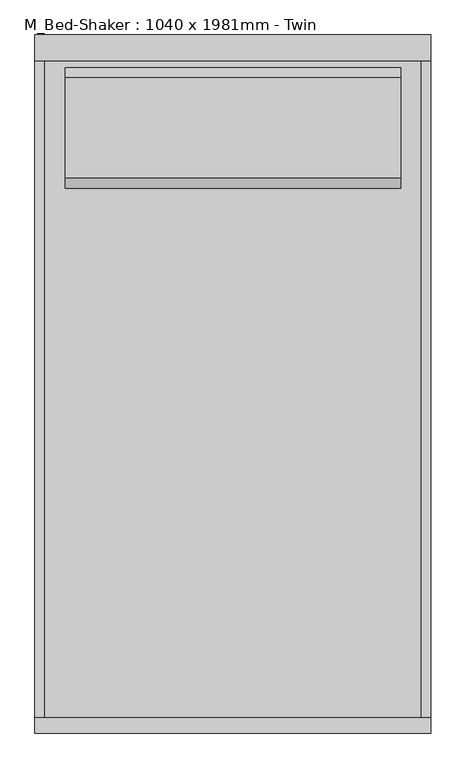
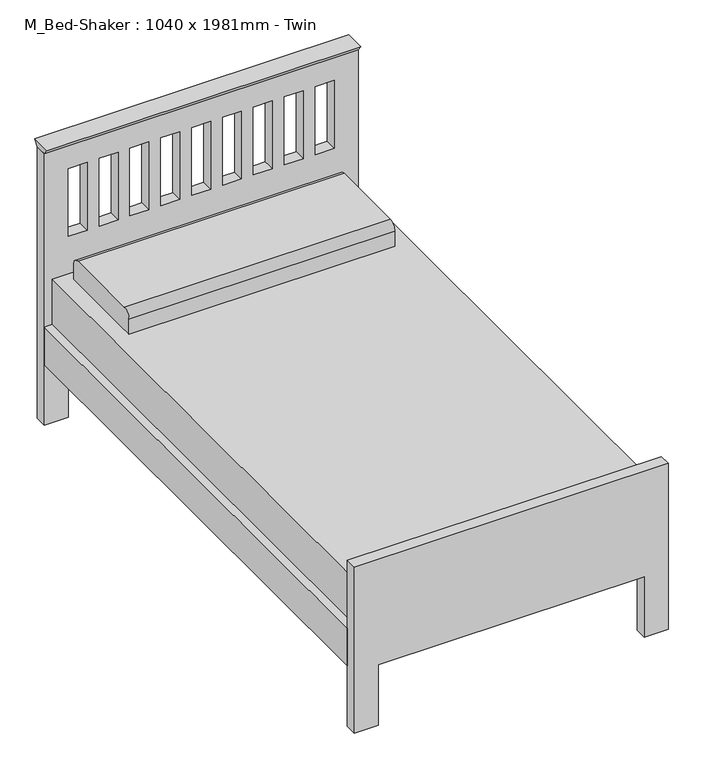
"""IFC4 building model written with IfcOpenShell, lengths in millimetres: furniture geometry, M_Bed-Shaker : 1040 x 1981mm - Twin."""

from ifc_helpers import new_model, si_unit, point, frame, frame_2d, origin, place, context, project, spatial, polyline, circle_curve, trimmed, segment, composite_curve, outline, extrude, source, transform, mapped, element, save


def m_bed_shaker_1040_x_1981mm_twin_8a9c4475(model_context):
    return source(origin(), model_context, "Body", "SweptSolid", [
        extrude(outline(polyline([(-38.1, 914.4), (-51.9545455, 933.45), (13.8545455, 933.45), (0.0, 914.4), (-38.1, 914.4)])), frame((-518.8365546, 0.0, 0.0), z_axis=(1.0, 0.0, 0.0), x_axis=(0.0, 1.0, 0.0)), (0.0, 0.0, 1.0), 1000.0533613),
        extrude(outline(composite_curve([segment(polyline([(-373.2486637, 482.6), (-373.2486637, 533.4)]), True, "CONTINUOUS"), segment(trimmed(circle_curve(frame_2d((-347.8486637, 533.4)), 25.4), [point((-373.2486637, 533.4))], [point((-347.8486637, 558.8))], False, "CARTESIAN"), True, "CONTINUOUS"), segment(polyline([(-347.8486637, 558.8), (-93.8486637, 558.8)]), True, "CONTINUOUS"), segment(trimmed(circle_curve(frame_2d((-93.8486637, 533.4)), 25.4), [point((-93.8486637, 558.8))], [point((-68.4486637, 533.4))], False, "CARTESIAN"), True, "CONTINUOUS"), segment(polyline([(-68.4486637, 533.4), (-68.4486637, 482.6), (-373.2486637, 482.6)]), True, "CONTINUOUS")], self_intersect=False)), frame((-442.85, 0.0, 0.0), z_axis=(1.0, 0.0, 0.0), x_axis=(0.0, 1.0, 0.0)), (0.0, 0.0, 1.0), 847.6),
        extrude(outline(polyline([(455.55, -38.1), (455.55, -1711.9), (-493.65, -1711.9), (-493.65, -38.1), (455.55, -38.1)])), frame((0.0, 0.0, 228.6), z_axis=(0.0, 0.0, 1.0), x_axis=(1.0, 0.0, 0.0)), (0.0, 0.0, 1.0), 254.0),
        extrude(outline(polyline([(455.55, -1711.9), (455.55, -38.1), (480.95, -38.1), (480.95, -1711.9), (455.55, -1711.9)])), frame((0.0, 0.0, 203.0994861), z_axis=(0.0, 0.0, 1.0), x_axis=(1.0, 0.0, 0.0)), (0.0, 0.0, 1.0), 127.0),
        extrude(outline(polyline([(-519.05, -1711.9), (-519.05, -38.1), (-493.65, -38.1), (-493.65, -1711.9), (-519.05, -1711.9)])), frame((0.0, 0.0, 203.5755296), z_axis=(0.0, 0.0, 1.0), x_axis=(1.0, 0.0, 0.0)), (0.0, 0.0, 1.0), 127.0),
        extrude(outline(polyline([(0.0, -442.85), (203.2, -442.85), (203.2, 404.75), (0.0, 404.75), (0.0, 480.95), (558.8, 480.95), (558.8, -519.05), (0.0, -519.05), (0.0, -442.85)])), frame((0.0, -1750.0, 0.0), z_axis=(0.0, 1.0, 0.0), x_axis=(0.0, 0.0, 1.0)), (0.0, 0.0, 1.0), 38.1),
        extrude(outline(polyline([(914.4, 481.2168067), (914.4, -518.8365546), (0.0, -518.8365546), (0.0, -442.85), (203.2, -442.85), (203.2, 404.75), (0.0, 404.75), (0.0, 481.2168067), (914.4, 481.2168067)]), holes=[polyline([(838.2, -382.5388889), (609.6, -382.5388889), (609.6, -442.85), (838.2, -442.85), (838.2, -382.5388889)]), polyline([(838.2, -284.1277778), (609.6, -284.1277778), (609.6, -344.4388889), (838.2, -344.4388889), (838.2, -284.1277778)]), polyline([(838.2, -185.7166667), (609.6, -185.7166667), (609.6, -246.0277778), (838.2, -246.0277778), (838.2, -185.7166667)]), polyline([(838.2, -87.3055556), (609.6, -87.3055556), (609.6, -147.6166667), (838.2, -147.6166667), (838.2, -87.3055556)]), polyline([(838.2, 109.5166667), (609.6, 109.5166667), (609.6, 49.2055556), (838.2, 49.2055556), (838.2, 109.5166667)]), polyline([(838.2, 207.9277778), (609.6, 207.9277778), (609.6, 147.6166667), (838.2, 147.6166667), (838.2, 207.9277778)]), polyline([(838.2, 306.3388889), (609.6, 306.3388889), (609.6, 246.0277778), (838.2, 246.0277778), (838.2, 306.3388889)]), polyline([(838.2, 404.75), (609.6, 404.75), (609.6, 344.4388889), (838.2, 344.4388889), (838.2, 404.75)]), polyline([(838.2, 11.1055556), (609.6, 11.1055556), (609.6, -49.2055556), (838.2, -49.2055556), (838.2, 11.1055556)])]), frame((0.0, -38.1, 0.0), z_axis=(0.0, 1.0, 0.0), x_axis=(0.0, 0.0, 1.0)), (0.0, 0.0, 1.0), 38.1),
    ])


if __name__ == "__main__":
    model = new_model("IFC4")
    model_context = context("Model", 3, world=origin())
    ifc_project = project(units=[si_unit("LENGTHUNIT", "METRE", prefix="MILLI")], contexts=[model_context])
    site = spatial("IfcSite", under=ifc_project)
    building = spatial("IfcBuilding", under=site)
    placement = place(None, origin())
    m_bed_shaker_1040_x_1981mm_twin_shape = m_bed_shaker_1040_x_1981mm_twin_8a9c4475(model_context)
    element("IfcFurniture", 1, ObjectType="M_Bed-Shaker : 1040 x 1981mm - Twin", at=placement, inside=building, context=model_context, shape_type="MappedRepresentation", body=[
        mapped(m_bed_shaker_1040_x_1981mm_twin_shape, transform((0.0, 0.0, 0.0), x_axis=(1.0, 0.0, 0.0), y_axis=(0.0, 1.0, 0.0), z_axis=(0.0, 0.0, 1.0))),
    ])
    save(model, "model.ifc")

# Revit data of these elements
# Type "M_Bed-Shaker : 1040 x 1981mm - Twin"
#   Length = 1.75 m
#   Width = 1 m
#   Frame Material = Birch
#   Mattress Material = Linen, White
# Element 1 (IfcFurniture, "M_Bed-Shaker : 1040 x 1981mm - Twin")
#   Materials on its faces: "Birch", "Linen, White"
# Materials
#   "Birch": class "Wood", colour RGB 224 178 126, transparency 0, Description = "Betula Alleghaniensis", Cost = 0
#   "Linen, White": class "Textile", colour RGB 247 247 239, transparency 0, Description = "Linen, white", Cost = 0
